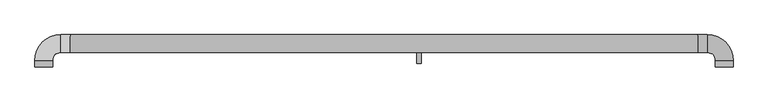
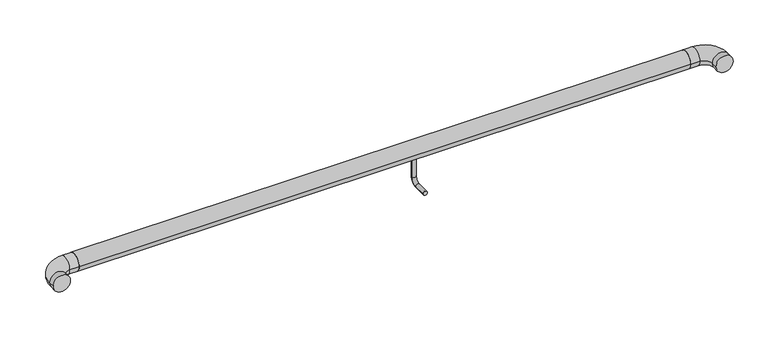
"""IFC4 building model written with IfcOpenShell, lengths in millimetres: railing geometry."""

from ifc_helpers import new_model, si_unit, point, frame, frame_2d, origin, place, context, project, spatial, circle_curve, ellipse_curve, trimmed, segment, composite_curve, outline, extrude, source, transform, mapped, element, save
from ifc_brep_helpers import plane_surface, cylinder_surface, revolved_surface, advanced_brep


def railing_c9e7f9bf(model_context):
    return source(origin(), model_context, "Body", "SolidModel", [
        extrude(outline(composite_curve([segment(trimmed(circle_curve(frame_2d((32228.1400611, 874.6)), 25.4), [point((32253.5400611, 874.6))], [point((32202.7400611, 874.6))], False, "CARTESIAN"), True, "CONTINUOUS"), segment(trimmed(circle_curve(frame_2d((32228.1400611, 874.6)), 25.4), [point((32202.7400611, 874.6))], [point((32253.5400611, 874.6))], False, "CARTESIAN"), True, "CONTINUOUS")], self_intersect=False)), frame((9766.6129185, 0.0, 0.0), z_axis=(1.0, 0.0, 0.0), x_axis=(0.0, 1.0, 0.0)), (0.0, 0.0, 1.0), 1800.0),
        advanced_brep(
        [(10760.2629185, 32228.1900611, 849.2), (10772.9629185, 32228.1900611, 849.2), (10760.2629185, 32228.1900611, 792.25), (10772.9629185, 32228.1900611, 792.25), (10772.9629185, 32209.1400611, 773.2), (10760.2629185, 32209.1400611, 773.2), (10760.2629185, 32170.7150611, 773.2), (10772.9629185, 32170.7150611, 773.2)],
        [
            (0, 1, circle_curve(frame((10766.6129185, 32228.1900611, 849.2), z_axis=(0.0, 0.0, 1.0), x_axis=(1.0, 0.0, 0.0)), 6.35)),
            (1, 0, circle_curve(frame((10766.6129185, 32228.1900611, 849.2), z_axis=(0.0, 0.0, 1.0), x_axis=(1.0, 0.0, 0.0)), 6.35)),
            (0, 2),
            (2, 3, circle_curve(frame((10766.6129185, 32228.1900611, 792.25), z_axis=(0.0, 0.0, 1.0), x_axis=(1.0, 0.0, 0.0)), 6.35)),
            (3, 1),
            (3, 2, circle_curve(frame((10766.6129185, 32228.1900611, 792.25), z_axis=(0.0, 0.0, 1.0), x_axis=(1.0, 0.0, 0.0)), 6.35)),
            (4, 3, circle_curve(frame((10772.9629185, 32209.1400611, 792.25), z_axis=(1.0, 0.0, 0.0), x_axis=(0.0, 1.0, 0.0)), 19.05)),
            (2, 5, circle_curve(frame((10760.2629185, 32209.1400611, 792.25), z_axis=(-1.0, 0.0, 0.0), x_axis=(0.0, 1.0, 0.0)), 19.05)),
            (5, 4, circle_curve(frame((10766.6129185, 32209.1400611, 773.2), z_axis=(0.0, 1.0, 0.0), x_axis=(1.0, 0.0, 0.0)), 6.35)),
            (4, 5, circle_curve(frame((10766.6129185, 32209.1400611, 773.2), z_axis=(0.0, 1.0, 0.0), x_axis=(1.0, 0.0, 0.0)), 6.35)),
            (6, 7, circle_curve(frame((10766.6129185, 32170.7150611, 773.2), z_axis=(0.0, -1.0, 0.0), x_axis=(1.0, 0.0, 0.0)), 6.35)),
            (7, 6, circle_curve(frame((10766.6129185, 32170.7150611, 773.2), z_axis=(0.0, -1.0, 0.0), x_axis=(1.0, 0.0, 0.0)), 6.35)),
            (5, 6),
            (7, 4),
        ],
        [
            plane_surface(frame((10772.9629185, 32228.1900611, 849.2), z_axis=(0.0, 0.0, 1.0), x_axis=(0.0, -1.0, 0.0))),
            cylinder_surface(frame((10766.6129185, 32228.1900611, 849.2), z_axis=(0.0, 0.0, 1.0), x_axis=(1.0, 0.0, 0.0)), 6.35),
            revolved_surface(trimmed(ellipse_curve(frame((10766.6129185, 32228.1900611, 792.25), z_axis=(0.0, 0.0, 1.0), x_axis=(1.0, 0.0, 0.0)), 6.35, 6.35), [point((10760.2629185, 32228.1900611, 792.25))], [point((10772.9629185, 32228.1900611, 792.25))], True, "CARTESIAN"), (10766.6129185, 32209.1400611, 792.25), (-1.0, 0.0, 0.0)),
            revolved_surface(trimmed(ellipse_curve(frame((10766.6129185, 32228.1900611, 792.25), z_axis=(0.0, 0.0, 1.0), x_axis=(1.0, 0.0, 0.0)), 6.35, 6.35), [point((10772.9629185, 32228.1900611, 792.25))], [point((10760.2629185, 32228.1900611, 792.25))], True, "CARTESIAN"), (10766.6129185, 32209.1400611, 792.25), (-1.0, 0.0, 0.0)),
            plane_surface(frame((10766.6129185, 32170.7150611, 766.85), z_axis=(0.0, -1.0, 0.0), x_axis=(1.0, 0.0, 0.0))),
            cylinder_surface(frame((10766.6129185, 32209.1400611, 773.2), z_axis=(0.0, 1.0, 0.0), x_axis=(1.0, 0.0, 0.0)), 6.35),
        ],
        [
            (0, [[1, 2]]),
            (1, [[-1, 3, 4, 5]]),
            (1, [[-2, -5, 6, -3]]),
            (2, [[7, -4, 8, 9]]),
            (3, [[-8, -6, -7, 10]]),
            (4, [[11, 12]]),
            (5, [[-9, 13, -12, 14]]),
            (5, [[-10, -14, -11, -13]]),
        ],
    ),
        advanced_brep(
        [(11566.6129185, 32202.7900611, 874.7), (11566.6129185, 32253.5900611, 874.7), (11594.1129185, 32202.7900611, 874.7), (11594.1129185, 32253.5900611, 874.7), (11668.0129185, 32179.6900611, 874.7), (11617.2129185, 32179.6900611, 874.7), (11617.2129185, 32161.1900611, 874.7), (11668.0129185, 32161.1900611, 874.7)],
        [
            (0, 1, circle_curve(frame((11566.6129185, 32228.1900611, 874.7), z_axis=(-1.0, 0.0, 0.0), x_axis=(0.0, 1.0, 0.0)), 25.4)),
            (1, 0, circle_curve(frame((11566.6129185, 32228.1900611, 874.7), z_axis=(-1.0, 0.0, 0.0), x_axis=(0.0, 1.0, 0.0)), 25.4)),
            (0, 2),
            (2, 3, circle_curve(frame((11594.1129185, 32228.1900611, 874.7), z_axis=(-1.0, 0.0, 0.0), x_axis=(0.0, 1.0, 0.0)), 25.4)),
            (3, 1),
            (3, 2, circle_curve(frame((11594.1129185, 32228.1900611, 874.7), z_axis=(-1.0, 0.0, 0.0), x_axis=(0.0, 1.0, 0.0)), 25.4)),
            (4, 3, circle_curve(frame((11594.1129185, 32179.6900611, 874.7), z_axis=(0.0, 0.0, 1.0), x_axis=(0.0, 1.0, 0.0)), 73.9)),
            (2, 5, circle_curve(frame((11594.1129185, 32179.6900611, 874.7), z_axis=(0.0, 0.0, -1.0), x_axis=(0.0, 1.0, 0.0)), 23.1)),
            (5, 4, circle_curve(frame((11642.6129185, 32179.6900611, 874.7), z_axis=(0.0, 1.0, 0.0), x_axis=(1.0, 0.0, 0.0)), 25.4)),
            (4, 5, circle_curve(frame((11642.6129185, 32179.6900611, 874.7), z_axis=(0.0, 1.0, 0.0), x_axis=(1.0, 0.0, 0.0)), 25.4)),
            (6, 7, circle_curve(frame((11642.6129185, 32161.1900611, 874.7), z_axis=(0.0, -1.0, 0.0), x_axis=(1.0, 0.0, 0.0)), 25.4)),
            (7, 6, circle_curve(frame((11642.6129185, 32161.1900611, 874.7), z_axis=(0.0, -1.0, 0.0), x_axis=(1.0, 0.0, 0.0)), 25.4)),
            (5, 6),
            (7, 4),
        ],
        [
            plane_surface(frame((11566.6129185, 32228.1900611, 874.7), z_axis=(-1.0, 0.0, 0.0), x_axis=(0.0, 0.0, 1.0))),
            cylinder_surface(frame((11566.6129185, 32228.1900611, 874.7), z_axis=(-1.0, 0.0, 0.0), x_axis=(0.0, 1.0, 0.0)), 25.4),
            revolved_surface(trimmed(ellipse_curve(frame((11594.1129185, 32228.1900611, 874.7), z_axis=(-1.0, 0.0, 0.0), x_axis=(0.0, 1.0, 0.0)), 25.4, 25.4), [point((11594.1129185, 32202.7900611, 874.7))], [point((11594.1129185, 32253.5900611, 874.7))], True, "CARTESIAN"), (11594.1129185, 32179.6900611, 874.7), (0.0, 0.0, -1.0)),
            revolved_surface(trimmed(ellipse_curve(frame((11594.1129185, 32228.1900611, 874.7), z_axis=(-1.0, 0.0, 0.0), x_axis=(0.0, 1.0, 0.0)), 25.4, 25.4), [point((11594.1129185, 32253.5900611, 874.7))], [point((11594.1129185, 32202.7900611, 874.7))], True, "CARTESIAN"), (11594.1129185, 32179.6900611, 874.7), (0.0, 0.0, -1.0)),
            plane_surface(frame((11642.6129185, 32161.1900611, 874.7), z_axis=(0.0, -1.0, 0.0), x_axis=(0.0, 0.0, 1.0))),
            cylinder_surface(frame((11642.6129185, 32179.6900611, 874.7), z_axis=(0.0, 1.0, 0.0), x_axis=(1.0, 0.0, 0.0)), 25.4),
        ],
        [
            (0, [[1, 2]]),
            (1, [[-1, 3, 4, 5]]),
            (1, [[-2, -5, 6, -3]]),
            (2, [[7, -4, 8, 9]]),
            (3, [[-8, -6, -7, 10]]),
            (4, [[11, 12]]),
            (5, [[-9, 13, -12, 14]]),
            (5, [[-10, -14, -11, -13]]),
        ],
    ),
        advanced_brep(
        [(9766.6129185, 32253.5900611, 874.7), (9766.6129185, 32202.7900611, 874.7), (9739.1129185, 32202.7900611, 874.7), (9739.1129185, 32253.5900611, 874.7), (9665.2129185, 32179.6900611, 874.7), (9716.0129185, 32179.6900611, 874.7), (9665.2129185, 32161.1900611, 874.7), (9716.0129185, 32161.1900611, 874.7)],
        [
            (0, 1, circle_curve(frame((9766.6129185, 32228.1900611, 874.7), z_axis=(1.0, 0.0, 0.0), x_axis=(0.0, -1.0, 0.0)), 25.4)),
            (1, 0, circle_curve(frame((9766.6129185, 32228.1900611, 874.7), z_axis=(1.0, 0.0, 0.0), x_axis=(0.0, -1.0, 0.0)), 25.4)),
            (1, 2),
            (2, 3, circle_curve(frame((9739.1129185, 32228.1900611, 874.7), z_axis=(1.0, 0.0, 0.0), x_axis=(0.0, -1.0, 0.0)), 25.4)),
            (3, 0),
            (3, 2, circle_curve(frame((9739.1129185, 32228.1900611, 874.7), z_axis=(1.0, 0.0, 0.0), x_axis=(0.0, -1.0, 0.0)), 25.4)),
            (4, 3, circle_curve(frame((9739.1129185, 32179.6900611, 874.7), z_axis=(0.0, 0.0, -1.0), x_axis=(0.0, 1.0, 0.0)), 73.9)),
            (2, 5, circle_curve(frame((9739.1129185, 32179.6900611, 874.7), z_axis=(0.0, 0.0, 1.0), x_axis=(0.0, 1.0, 0.0)), 23.1)),
            (5, 4, circle_curve(frame((9690.6129185, 32179.6900611, 874.7), z_axis=(0.0, 1.0, 0.0), x_axis=(1.0, 0.0, 0.0)), 25.4)),
            (4, 5, circle_curve(frame((9690.6129185, 32179.6900611, 874.7), z_axis=(0.0, 1.0, 0.0), x_axis=(1.0, 0.0, 0.0)), 25.4)),
            (6, 7, circle_curve(frame((9690.6129185, 32161.1900611, 874.7), z_axis=(0.0, -1.0, 0.0), x_axis=(1.0, 0.0, 0.0)), 25.4)),
            (7, 6, circle_curve(frame((9690.6129185, 32161.1900611, 874.7), z_axis=(0.0, -1.0, 0.0), x_axis=(1.0, 0.0, 0.0)), 25.4)),
            (5, 7),
            (6, 4),
        ],
        [
            plane_surface(frame((9766.6129185, 32228.1900611, 874.7), z_axis=(1.0, 0.0, 0.0), x_axis=(0.0, 0.0, 1.0))),
            cylinder_surface(frame((9766.6129185, 32228.1900611, 874.7), z_axis=(1.0, 0.0, 0.0), x_axis=(0.0, -1.0, 0.0)), 25.4),
            revolved_surface(trimmed(ellipse_curve(frame((9739.1129185, 32228.1900611, 874.7), z_axis=(1.0, 0.0, 0.0), x_axis=(0.0, -1.0, 0.0)), 25.4, 25.4), [point((9739.1129185, 32202.7900611, 874.7))], [point((9739.1129185, 32253.5900611, 874.7))], True, "CARTESIAN"), (9739.1129185, 32179.6900611, 874.7), (0.0, 0.0, 1.0)),
            revolved_surface(trimmed(ellipse_curve(frame((9739.1129185, 32228.1900611, 874.7), z_axis=(1.0, 0.0, 0.0), x_axis=(0.0, -1.0, 0.0)), 25.4, 25.4), [point((9739.1129185, 32253.5900611, 874.7))], [point((9739.1129185, 32202.7900611, 874.7))], True, "CARTESIAN"), (9739.1129185, 32179.6900611, 874.7), (0.0, 0.0, 1.0)),
            plane_surface(frame((9690.6129185, 32161.1900611, 874.7), z_axis=(0.0, -1.0, 0.0), x_axis=(0.0, 0.0, 1.0))),
            cylinder_surface(frame((9690.6129185, 32179.6900611, 874.7), z_axis=(0.0, 1.0, 0.0), x_axis=(1.0, 0.0, 0.0)), 25.4),
        ],
        [
            (0, [[1, 2]]),
            (1, [[-2, 3, 4, 5]]),
            (1, [[-1, -5, 6, -3]]),
            (2, [[7, -4, 8, 9]]),
            (3, [[-8, -6, -7, 10]]),
            (4, [[11, 12]]),
            (5, [[-9, 13, -11, 14]]),
            (5, [[-10, -14, -12, -13]]),
        ],
    ),
    ])


if __name__ == "__main__":
    model = new_model("IFC4")
    model_context = context("Model", 3, world=origin())
    ifc_project = project(units=[si_unit("LENGTHUNIT", "METRE", prefix="MILLI")], contexts=[model_context])
    site = spatial("IfcSite", under=ifc_project)
    building = spatial("IfcBuilding", under=site)
    placement = place(None, origin())
    railing_shape = railing_c9e7f9bf(model_context)
    element("IfcRailing", 1, at=placement, inside=building, context=model_context, shape_type="MappedRepresentation", body=[
        mapped(railing_shape, transform((0.0, 0.0, 0.0), x_axis=(1.0, 0.0, 0.0), y_axis=(0.0, 1.0, 0.0), z_axis=(0.0, 0.0, 1.0))),
    ])
    save(model, "model.ifc")

# Revit data of these elements
# Element 1 (IfcRailing)
#   Materials on its faces: "Ferro - Pintura Esmalte"
# Materials
#   "Ferro - Pintura Esmalte": class "Pintura", colour RGB 255 255 255, transparency 0, Cost = 0
